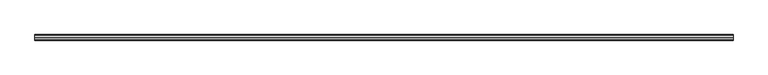
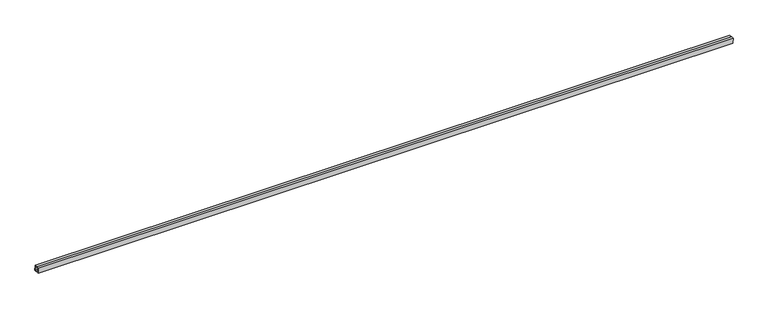
"""IFC4 building model written with IfcOpenShell, lengths in millimetres: proxy geometry, Inner panel:Inner panel:1:Inner panel:1 : Inner panel:Inner panel:300324:2:Inner panel:1:Inner panel:1 : Inner panel:Inner panel:300324:2 : Inner panel:Inner panel:1:Inner panel:1 : Inner panel:Inner panel:300324:300043:54 : Inner panel:Inner panel:1:Inner panel:1 : Inner panel:Inner panel:300324:2:Inner panel:1:Inner panel:1 : Inner panel:Inner panel:300324:2 : Inner panel:Inner panel:1:Inner panel:1 : Inner panel:Inner panel:300324:300043:308120."""

from ifc_helpers import new_model, si_unit, frame, origin, place, context, project, spatial, polyline, outline, extrude, source, transform, mapped, element, save


def generic_models_14f8ca5c(model_context):
    return source(origin(), model_context, "Body", "SweptSolid", [
        extrude(outline(polyline([(-581211.0091179, 3857.8017792), (-581192.7686948, 3858.5617968), (-581191.182571, 3820.4948267), (-581229.2495411, 3818.908703), (-581230.8356649, 3856.9756731), (-581212.5952417, 3857.7356907), (-581212.496109, 3855.3565051), (-581228.3573465, 3854.6956202), (-581226.9694882, 3821.3870213), (-581193.6608894, 3822.7748796), (-581195.0487477, 3856.0834785), (-581210.9099852, 3855.4225936), (-581211.0091179, 3857.8017792)])), frame((659327.2367238, 0.0, 0.0), z_axis=(1.0, 0.0, 0.0), x_axis=(0.0, 1.0, 0.0)), (0.0, 0.0, 1.0), 4876.8),
    ])


if __name__ == "__main__":
    model = new_model("IFC4")
    model_context = context("Model", 3, world=origin())
    ifc_project = project(units=[si_unit("LENGTHUNIT", "METRE", prefix="MILLI")], contexts=[model_context])
    site = spatial("IfcSite", under=ifc_project)
    building = spatial("IfcBuilding", under=site)
    placement = place(None, origin())
    generic_models_shape = generic_models_14f8ca5c(model_context)
    element("IfcBuildingElementProxy", 1, Name="Inner panel:Inner panel:1:Inner panel:1 : Inner panel:Inner panel:300324:2:Inner panel:1:Inner panel:1 : Inner panel:Inner panel:300324:2 : Inner panel:Inner panel:1:Inner panel:1 : Inner panel:Inner panel:300324:300043:54 : Inner panel:Inner panel:1:Inner panel:1 : Inner panel:Inner panel:300324:2:Inner panel:1:Inner panel:1 : Inner panel:Inner panel:300324:2 : Inner panel:Inner panel:1:Inner panel:1 : Inner panel:Inner panel:300324:300043:308120", ObjectType="Inner panel:Inner panel:1:Inner panel:1 : Inner panel:Inner panel:300324:2:Inner panel:1:Inner panel:1 : Inner panel:Inner panel:300324:2 : Inner panel:Inner panel:1:Inner panel:1 : Inner panel:Inner panel:300324:300043:54 : Inner panel:Inner panel:1:Inner panel:1 : Inner panel:Inner panel:300324:2:Inner panel:1:Inner panel:1 : Inner panel:Inner panel:300324:2 : Inner panel:Inner panel:1:Inner panel:1 : Inner panel:Inner panel:300324:300043:308120", at=placement, inside=building, context=model_context, shape_type="MappedRepresentation", body=[
        mapped(generic_models_shape, transform((0.0, 0.0, 0.0), x_axis=(1.0, 0.0, 0.0), y_axis=(0.0, 1.0, 0.0), z_axis=(0.0, 0.0, 1.0))),
    ])
    save(model, "model.ifc")

# Revit data of these elements
# Type "Inner panel:Inner panel:1:Inner panel:1 : Inner panel:Inner panel:300324:2:Inner panel:1:Inner panel:1 : Inner panel:Inner panel:300324:2 : Inner panel:Inner panel:1:Inner panel:1 : Inner panel:Inner panel:300324:300043:54 : Inner panel:Inner panel:1:Inner panel:1 : Inner panel:Inner panel:300324:2:Inner panel:1:Inner panel:1 : Inner panel:Inner panel:300324:2 : Inner panel:Inner panel:1:Inner panel:1 : Inner panel:Inner panel:300324:300043:308120"
#   NameOverride = "Inner panel:Inner panel:1:Inner panel:1 : Inner panel:Inner panel:300324:2:Inner panel:1:Inner panel:1 : Inner panel:Inner panel:300324:2 : Inner panel:Inner panel:1:Inner panel:1 : Inner panel:Inner panel:300324:300043:308120"
#   ObjectTypeOverride = "Inner panel:1:Inner panel:1 : Inner panel:Inner panel:300324:2 : Inner panel:Inner panel:1:Inner panel:1 : Inner panel:Inner panel:300324:300043"
#   Reference = "Inner panel"
#   Tag = "308120"
# Element 1 (IfcBuildingElementProxy, "Inner panel:Inner panel:1:Inner panel:1 : Inner panel:Inner panel:300324:2:Inner panel:1:Inner panel:1 : Inner panel:Inner panel:300324:2 : Inner panel:Inner panel:1:Inner panel:1 : Inner panel:Inner panel:300324:300043:54 : Inner panel:Inner panel:1:Inner panel:1 : Inner panel:Inner panel:300324:2:Inner panel:1:Inner panel:1 : Inner panel:Inner panel:300324:2 : Inner panel:Inner panel:1:Inner panel:1 : Inner panel:Inner panel:300324:300043:308120")
#   Materials on its faces: "1 1/2\" X 1 1/2\" SPLIT-SEAM SQUARE TUBING (~24\" CANTILEVER FROM C.L. OF GLULAM)"
# Materials
#   "1 1/2\" X 1 1/2\" SPLIT-SEAM SQUARE TUBING (~24\" CANTILEVER FROM C.L. OF GLULAM)": class "Unassigned", colour RGB 202 201 200, transparency 0, Cost = 0
